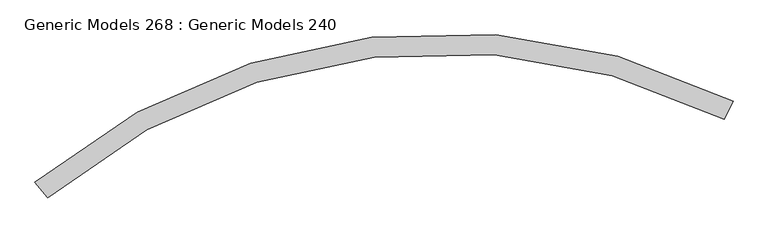
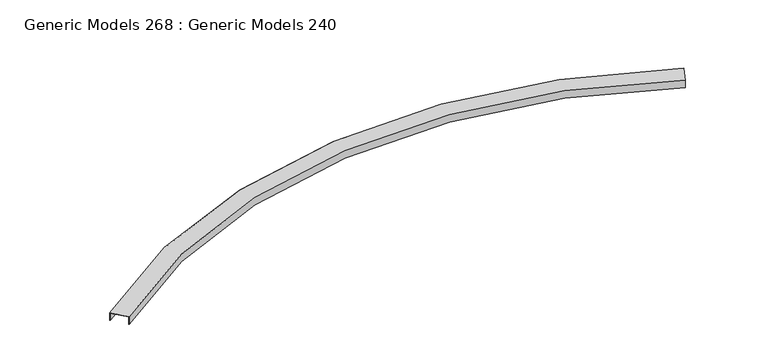
"""IFC4 building model written with IfcOpenShell, lengths in millimetres: proxy geometry, Generic Models 268 : Generic Models 240."""

from ifc_helpers import new_model, si_unit, frame, origin, place, context, project, spatial, polyline, circle_curve, source, transform, mapped, element, save
from ifc_brep_helpers import plane_surface, cylinder_surface, revolved_surface, advanced_brep


def generic_models_268_generic_models_240_5ae7cd61(model_context):
    return source(origin(), model_context, "Body", "AdvancedBrep", [
        advanced_brep(
        [(443.8139737, -22599.4854672, 781.05), (443.8139737, -22599.4854672, 739.775), (444.5265897, -22598.0668994, 739.775), (444.5265897, -22598.0668994, 779.4625), (484.4330886, -22518.6271024, 779.4625), (484.4330886, -22518.6271024, 739.775), (485.1457047, -22517.2085346, 739.775), (485.1457047, -22517.2085346, 781.05), (-2656.3078884, -22959.7283673, 781.05), (-2715.4051403, -22889.1215656, 781.05), (-2715.4051403, -22889.1215656, 739.775), (-2714.3862222, -22890.3389242, 739.775), (-2714.3862222, -22890.3389242, 779.4625), (-2657.3268065, -22958.5110086, 779.4625), (-2657.3268065, -22958.5110086, 739.775), (-2656.3078884, -22959.7283673, 739.775)],
        [
            (0, 1),
            (1, 2),
            (2, 3),
            (3, 4),
            (4, 5),
            (5, 6),
            (6, 7),
            (7, 0),
            (8, 9),
            (9, 10),
            (10, 11),
            (11, 12),
            (12, 13),
            (13, 14),
            (14, 15),
            (15, 8),
            (15, 1, circle_curve(frame((-832.04683, -25139.2753781, 739.775), z_axis=(0.0, 0.0, -1.0), x_axis=(0.44889200092737946, 0.8935860179654858, 0.0)), 2842.244462)),
            (0, 8, circle_curve(frame((-832.04683, -25139.2753781, 781.05), z_axis=(0.0, 0.0, 1.0), x_axis=(0.44889200092737946, 0.8935860179654858, 0.0)), 2842.244462)),
            (14, 2, circle_curve(frame((-832.04683, -25139.2753781, 739.775), z_axis=(0.0, 0.0, -1.0), x_axis=(0.44889200092737946, 0.8935860179654858, 0.0)), 2843.831962)),
            (13, 3, circle_curve(frame((-832.04683, -25139.2753781, 779.4625), z_axis=(0.0, 0.0, -1.0), x_axis=(0.44889200092737946, 0.8935860179654858, 0.0)), 2843.831962)),
            (12, 4, circle_curve(frame((-832.04683, -25139.2753781, 779.4625), z_axis=(0.0, 0.0, -1.0), x_axis=(0.44889200092737946, 0.8935860179654858, 0.0)), 2932.731962)),
            (11, 5, circle_curve(frame((-832.04683, -25139.2753781, 739.775), z_axis=(0.0, 0.0, -1.0), x_axis=(0.44889200092737946, 0.8935860179654858, 0.0)), 2932.731962)),
            (10, 6, circle_curve(frame((-832.04683, -25139.2753781, 739.775), z_axis=(0.0, 0.0, -1.0), x_axis=(0.44889200092737946, 0.8935860179654858, 0.0)), 2934.319462)),
            (9, 7, circle_curve(frame((-832.04683, -25139.2753781, 781.05), z_axis=(0.0, 0.0, -1.0), x_axis=(0.44889200092737946, 0.8935860179654858, 0.0)), 2934.319462)),
        ],
        [
            plane_surface(frame((536.1759889, -22415.6251953, 82.55), z_axis=(0.8935860179654859, -0.4488920009273796, 0.0), x_axis=(0.0, 0.0, -1.0))),
            plane_surface(frame((-2788.3696518, -22801.9467711, 82.55), z_axis=(-0.7668400941499618, -0.6418381961242863, 0.0), x_axis=(0.0, 0.0, -1.0))),
            revolved_surface(polyline([(443.81397367194313, -22599.485467216964, 781.05), (443.81397367194313, -22599.485467216964, 739.775)]), (-832.04683, -25139.2753781, 82.55), (0.0, 0.0, 1.0)),
            plane_surface(frame((-832.04683, -25139.2753781, 739.775), z_axis=(0.0, 0.0, -1.0000000000000002), x_axis=(0.4488920009273795, 0.8935860179654859, 0.0))),
            cylinder_surface(frame((-832.04683, -25139.2753781, 82.55), z_axis=(0.0, 0.0, 1.0), x_axis=(0.44889200092737946, 0.8935860179654858, 0.0)), 2843.831962),
            plane_surface(frame((-832.04683, -25139.2753781, 779.4625), z_axis=(0.0, 0.0, -1.0000000000000002), x_axis=(0.4488920009273795, 0.8935860179654859, 0.0))),
            revolved_surface(polyline([(484.4330886058592, -22518.627102416314, 779.4625), (484.4330886058592, -22518.627102416314, 739.775)]), (-832.04683, -25139.2753781, 82.55), (0.0, 0.0, 1.0)),
            cylinder_surface(frame((-832.04683, -25139.2753781, 82.55), z_axis=(0.0, 0.0, 1.0), x_axis=(0.44889200092737946, 0.8935860179654858, 0.0)), 2934.319462),
            plane_surface(frame((-832.04683, -25139.2753781, 781.05), z_axis=(0.0, 0.0, 1.0000000000000002), x_axis=(0.4488920009273795, 0.8935860179654859, 0.0))),
        ],
        [
            (0, [[1, 2, 3, 4, 5, 6, 7, 8]]),
            (1, [[9, 10, 11, 12, 13, 14, 15, 16]]),
            (2, [[17, -1, 18, -16]]),
            (3, [[19, -2, -17, -15]]),
            (4, [[20, -3, -19, -14]]),
            (5, [[21, -4, -20, -13]]),
            (6, [[22, -5, -21, -12]]),
            (3, [[23, -6, -22, -11]]),
            (7, [[24, -7, -23, -10]]),
            (8, [[-18, -8, -24, -9]]),
        ],
    ),
    ])


if __name__ == "__main__":
    model = new_model("IFC4")
    model_context = context("Model", 3, world=origin())
    ifc_project = project(units=[si_unit("LENGTHUNIT", "METRE", prefix="MILLI")], contexts=[model_context])
    site = spatial("IfcSite", under=ifc_project)
    building = spatial("IfcBuilding", under=site)
    placement = place(None, origin())
    generic_models_268_generic_models_240_shape = generic_models_268_generic_models_240_5ae7cd61(model_context)
    element("IfcBuildingElementProxy", 1, Name="Generic Models 268 : Generic Models 240", ObjectType="Generic Models 268 : Generic Models 240", at=placement, inside=building, context=model_context, shape_type="MappedRepresentation", body=[
        mapped(generic_models_268_generic_models_240_shape, transform((0.0, 0.0, 0.0), x_axis=(1.0, 0.0, 0.0), y_axis=(0.0, 1.0, 0.0), z_axis=(0.0, 0.0, 1.0))),
    ])
    save(model, "model.ifc")
